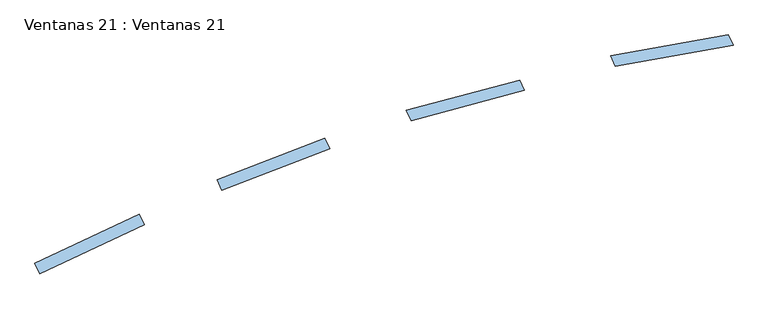
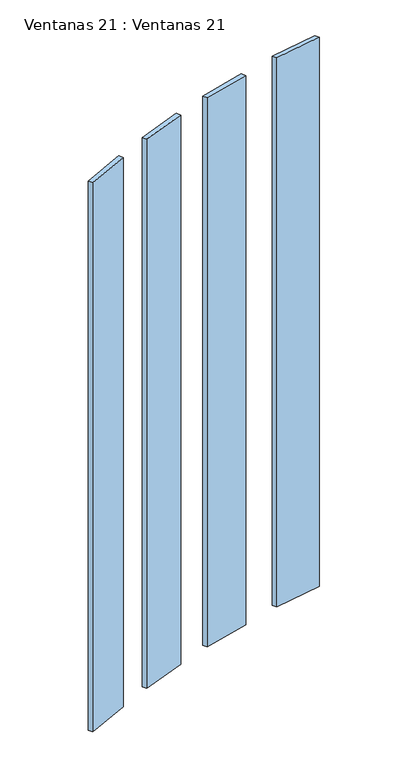
"""IFC4 building model written with IfcOpenShell, lengths in millimetres: window geometry, Ventanas 21 : Ventanas 21."""

from ifc_helpers import new_model, si_unit, frame, origin, place, context, project, spatial, polyline, outline, extrude, source, transform, mapped, element, save


def ventanas_21_ventanas_21_fa48c21e(model_context):
    return source(origin(), model_context, "Body", "SweptSolid", [
        extrude(outline(polyline([(834.168643, 6839.7095084), (842.6210082, 6821.5833527), (661.3594508, 6737.0597003), (652.9070855, 6755.1858561), (834.168643, 6839.7095084)])), frame((0.0, 0.0, 6038.2783034), z_axis=(0.0, 0.0, 1.0), x_axis=(1.0, 0.0, 0.0)), (0.0, 0.0, 1.0), 2493.4673348),
        extrude(outline(polyline([(1155.8252083, 6971.4344922), (1164.2775736, 6953.3083364), (977.1055466, 6881.4597269), (968.6531814, 6899.5858827), (1155.8252083, 6971.4344922)])), frame((0.0, 0.0, 6038.2783034), z_axis=(0.0, 0.0, 1.0), x_axis=(1.0, 0.0, 0.0)), (0.0, 0.0, 1.0), 2493.4673348),
        extrude(outline(polyline([(1493.3322499, 7072.664686), (1501.7846151, 7054.5385303), (1305.6192573, 7001.9761811), (1297.1668921, 7020.1023368), (1493.3322499, 7072.664686)])), frame((0.0, 0.0, 6038.2783034), z_axis=(0.0, 0.0, 1.0), x_axis=(1.0, 0.0, 0.0)), (0.0, 0.0, 1.0), 2493.4673348),
        extrude(outline(polyline([(1855.027521, 7150.8979931), (1863.4798863, 7132.7718374), (1659.5702845, 7096.8170729), (1651.1179192, 7114.9432287), (1855.027521, 7150.8979931)])), frame((0.0, 0.0, 6038.2783034), z_axis=(0.0, 0.0, 1.0), x_axis=(1.0, 0.0, 0.0)), (0.0, 0.0, 1.0), 2493.4673348),
    ])


if __name__ == "__main__":
    model = new_model("IFC4")
    model_context = context("Model", 3, world=origin())
    ifc_project = project(units=[si_unit("LENGTHUNIT", "METRE", prefix="MILLI")], contexts=[model_context])
    site = spatial("IfcSite", under=ifc_project)
    building = spatial("IfcBuilding", under=site)
    placement = place(None, origin())
    ventanas_21_ventanas_21_shape = ventanas_21_ventanas_21_fa48c21e(model_context)
    element("IfcWindow", 1, ObjectType="Ventanas 21 : Ventanas 21", at=placement, inside=building, context=model_context, shape_type="MappedRepresentation", body=[
        mapped(ventanas_21_ventanas_21_shape, transform((0.0, 0.0, 0.0), x_axis=(1.0, 0.0, 0.0), y_axis=(0.0, 1.0, 0.0), z_axis=(0.0, 0.0, 1.0))),
    ])
    save(model, "model.ifc")

# Revit data of these elements
# Type "Ventanas 21 : Ventanas 21"
#   Type Mark = "49"
# Element 1 (IfcWindow, "Ventanas 21 : Ventanas 21")
#   Materials on its faces: "VIDRIO"
# Materials
#   "VIDRIO": class "Genérico", colour RGB 120 120 120, transparency 0, Cost = 0
